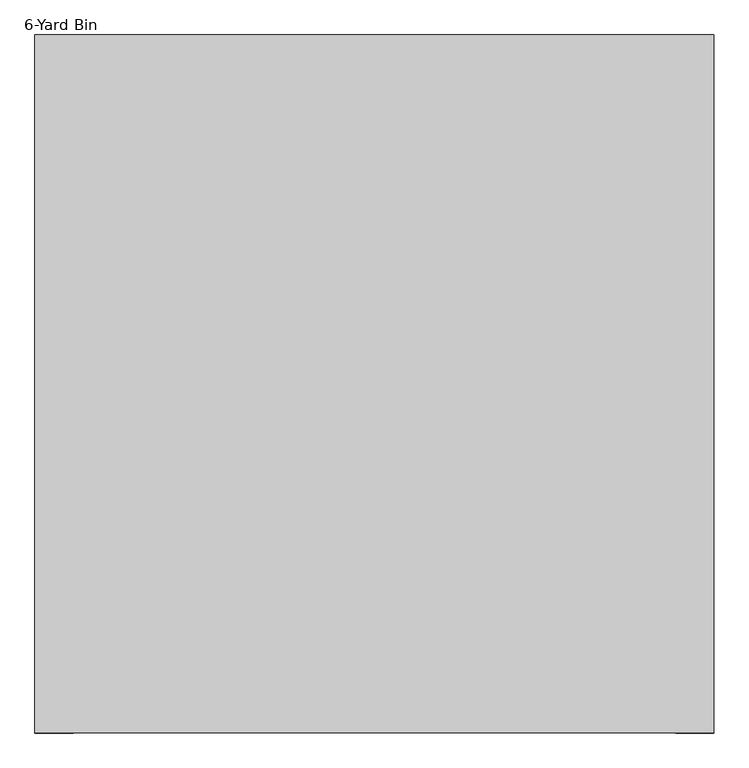
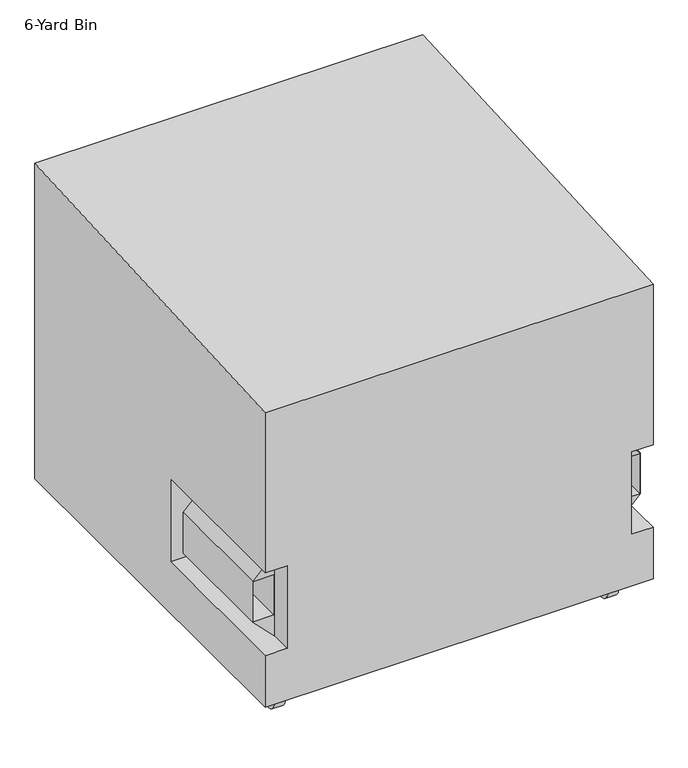
"""IFC4 building model written with IfcOpenShell, lengths in millimetres: proxy geometry, 323323 - Site Trash and Litter Receptacles - Dumpsters : 6-Yard Bin."""

from ifc_helpers import new_model, si_unit, point, frame, frame_2d, origin, place, context, project, spatial, circle_curve, trimmed, segment, composite_curve, outline, extrude, faceted_brep, source, transform, mapped, element, save


def proxy_6_yard_bin_48c06d3c(model_context):
    return source(origin(), model_context, "Body", "SolidModel", [
        faceted_brep([(901.7, 927.1, 127.0), (901.7, 927.1, 1676.4), (901.7, -927.1, 1574.8), (901.7, -927.1, 787.4), (901.7, -825.5, 787.4), (901.7, -266.7, 787.4), (901.7, -165.1, 787.4), (901.7, -165.1, 381.0), (901.7, -266.7, 381.0), (901.7, -825.5, 381.0), (901.7, -927.1, 381.0), (901.7, -927.1, 127.0), (901.7, -825.5, 685.8), (901.7, -825.5, 482.6), (901.7, -266.7, 482.6), (901.7, -266.7, 685.8), (-901.7, 927.1, 127.0), (-901.7, -927.1, 127.0), (-901.7, -927.1, 381.0), (-901.7, -825.5, 381.0), (-901.7, -266.7, 381.0), (-901.7, -165.1, 381.0), (-901.7, -165.1, 787.4), (-901.7, -266.7, 787.4), (-901.7, -825.5, 787.4), (-901.7, -927.1, 787.4), (-901.7, -927.1, 1574.8), (-901.7, 927.1, 1676.4), (-901.7, -825.5, 482.6), (-901.7, -825.5, 685.8), (-901.7, -266.7, 685.8), (-901.7, -266.7, 482.6), (-800.1, -927.1, 787.4), (-800.1, -927.1, 381.0), (800.1, -927.1, 381.0), (800.1, -927.1, 787.4), (800.1, -165.1, 787.4), (800.1, -165.1, 381.0), (-800.1, -165.1, 787.4), (-800.1, -165.1, 381.0), (-800.1, -266.7, 787.4), (-800.1, -825.5, 787.4), (-800.1, -825.5, 381.0), (-800.1, -266.7, 381.0), (-898.525, -825.5, 485.775), (-803.275, -825.5, 485.775), (-803.275, -266.7, 485.775), (-898.525, -266.7, 485.775), (-803.275, -825.5, 682.625), (-803.275, -266.7, 682.625), (-898.525, -825.5, 682.625), (-898.525, -266.7, 682.625), (800.1, -825.5, 787.4), (800.1, -266.7, 787.4), (800.1, -266.7, 381.0), (800.1, -825.5, 381.0), (898.525, -825.5, 485.775), (898.525, -825.5, 682.625), (898.525, -266.7, 682.625), (898.525, -266.7, 485.775), (803.275, -825.5, 682.625), (803.275, -266.7, 682.625), (803.275, -825.5, 485.775), (803.275, -266.7, 485.775)], [[[0, 1, 2, 3, 4, 5, 6, 7, 8, 9, 10, 11]], [[12, 13, 14, 15]], [[16, 17, 18, 19, 20, 21, 22, 23, 24, 25, 26, 27]], [[28, 29, 30, 31]], [[1, 0, 16, 27]], [[2, 1, 27, 26]], [[2, 26, 25, 32, 33, 18, 17, 11, 10, 34, 35, 3]], [[0, 11, 17, 16]], [[6, 36, 37, 7]], [[38, 22, 21, 39]], [[22, 38, 40, 41, 32, 25, 24, 23]], [[29, 41, 40, 30]], [[42, 28, 31, 43]], [[39, 21, 20, 19, 18, 33, 42, 43]], [[44, 45, 46, 47]], [[45, 48, 49, 46]], [[48, 50, 51, 49]], [[50, 44, 47, 51]], [[52, 12, 15, 53]], [[36, 6, 5, 4, 3, 35, 52, 53]], [[7, 37, 54, 55, 34, 10, 9, 8]], [[13, 55, 54, 14]], [[56, 57, 58, 59]], [[57, 60, 61, 58]], [[60, 62, 63, 61]], [[62, 56, 59, 63]], [[41, 42, 33, 32]], [[42, 41, 29, 28], [45, 44, 50, 48]], [[55, 52, 35, 34]], [[52, 55, 13, 12], [57, 56, 62, 60]], [[43, 40, 38, 39]], [[40, 43, 31, 30], [47, 46, 49, 51]], [[37, 36, 53, 54]], [[54, 53, 15, 14], [59, 58, 61, 63]]]),
        extrude(outline(composite_curve([segment(trimmed(circle_curve(frame_2d((-774.7, 50.8)), 50.8), [point((-825.5, 50.8))], [point((-723.9, 50.8))], False, "CARTESIAN"), True, "CONTINUOUS"), segment(trimmed(circle_curve(frame_2d((-774.7, 50.8)), 50.8), [point((-723.9, 50.8))], [point((-825.5, 50.8))], False, "CARTESIAN"), True, "CONTINUOUS")], self_intersect=False)), frame((749.3, 0.0, 0.0), z_axis=(1.0, 0.0, 0.0), x_axis=(0.0, 1.0, 0.0)), (0.0, 0.0, 1.0), 50.8),
        extrude(outline(composite_curve([segment(trimmed(circle_curve(frame_2d((774.7, 50.8)), 50.8), [point((723.9, 50.8))], [point((825.5, 50.8))], False, "CARTESIAN"), True, "CONTINUOUS"), segment(trimmed(circle_curve(frame_2d((774.7, 50.8)), 50.8), [point((825.5, 50.8))], [point((723.9, 50.8))], False, "CARTESIAN"), True, "CONTINUOUS")], self_intersect=False)), frame((749.3, 0.0, 0.0), z_axis=(1.0, 0.0, 0.0), x_axis=(0.0, 1.0, 0.0)), (0.0, 0.0, 1.0), 50.8),
        extrude(outline(composite_curve([segment(trimmed(circle_curve(frame_2d((774.7, 50.8)), 50.8), [point((723.9, 50.8))], [point((825.5, 50.8))], False, "CARTESIAN"), True, "CONTINUOUS"), segment(trimmed(circle_curve(frame_2d((774.7, 50.8)), 50.8), [point((825.5, 50.8))], [point((723.9, 50.8))], False, "CARTESIAN"), True, "CONTINUOUS")], self_intersect=False)), frame((-800.1, 0.0, 0.0), z_axis=(1.0, 0.0, 0.0), x_axis=(0.0, 1.0, 0.0)), (0.0, 0.0, 1.0), 50.8),
        extrude(outline(composite_curve([segment(trimmed(circle_curve(frame_2d((-774.7, 50.8)), 50.8), [point((-825.5, 50.8))], [point((-723.9, 50.8))], False, "CARTESIAN"), True, "CONTINUOUS"), segment(trimmed(circle_curve(frame_2d((-774.7, 50.8)), 50.8), [point((-723.9, 50.8))], [point((-825.5, 50.8))], False, "CARTESIAN"), True, "CONTINUOUS")], self_intersect=False)), frame((-800.1, 0.0, 0.0), z_axis=(1.0, 0.0, 0.0), x_axis=(0.0, 1.0, 0.0)), (0.0, 0.0, 1.0), 50.8),
    ])


if __name__ == "__main__":
    model = new_model("IFC4")
    model_context = context("Model", 3, world=origin())
    ifc_project = project(units=[si_unit("LENGTHUNIT", "METRE", prefix="MILLI")], contexts=[model_context])
    site = spatial("IfcSite", under=ifc_project)
    building = spatial("IfcBuilding", under=site)
    placement = place(None, origin())
    proxy_6_yard_bin_shape = proxy_6_yard_bin_48c06d3c(model_context)
    element("IfcBuildingElementProxy", 1, Name="323323 - Site Trash and Litter Receptacles - Dumpsters : 6-Yard Bin", ObjectType="323323 - Site Trash and Litter Receptacles - Dumpsters : 6-Yard Bin", at=placement, inside=building, context=model_context, shape_type="MappedRepresentation", body=[
        mapped(proxy_6_yard_bin_shape, transform((0.0, 0.0, 0.0), x_axis=(1.0, 0.0, 0.0), y_axis=(0.0, 1.0, 0.0), z_axis=(0.0, 0.0, 1.0))),
    ])
    save(model, "model.ifc")

# Revit data of these elements
# Type "323323 - Site Trash and Litter Receptacles - Dumpsters : 6-Yard Bin"
#   WIDTH = 5' - 11"
#   HEIGHT - REAR = 5' - 6"
#   HEIGHT - FRONT = 5' - 2"
#   DEPTH = 6' - 1"
#   Material = 6 YARD DUMPSTER
# Element 1 (IfcBuildingElementProxy, "323323 - Site Trash and Litter Receptacles - Dumpsters : 6-Yard Bin")
#   Materials on its faces: "6 YARD DUMPSTER"
# Materials
#   "6 YARD DUMPSTER": class "Unassigned", colour RGB 202 224 201, transparency 0, Comments = "Rendering appearance not upgraded ", Cost = 0
